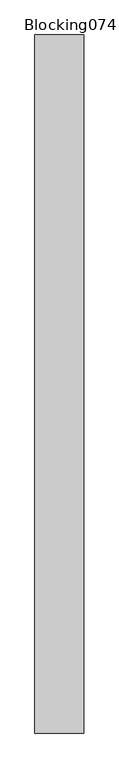
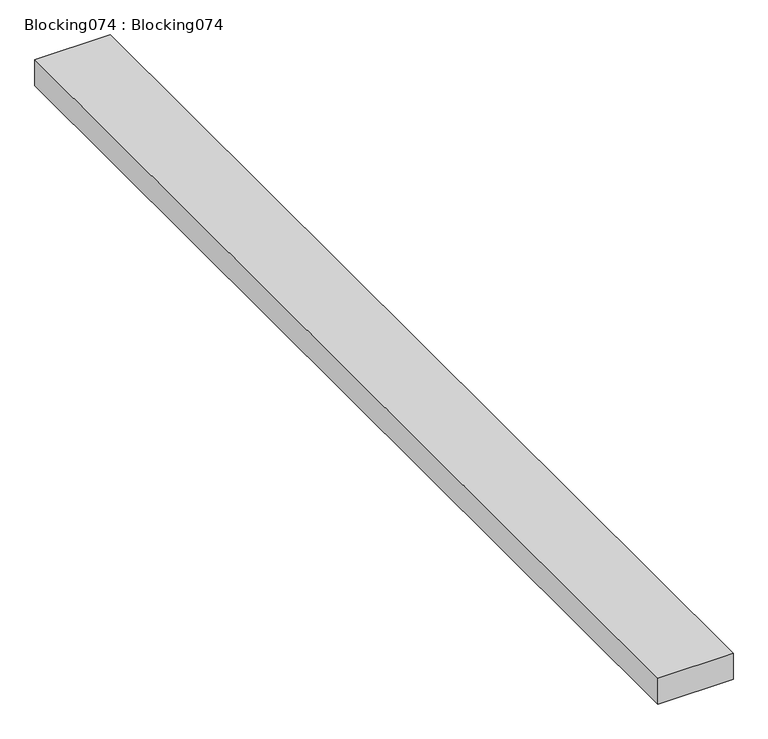
"""IFC4 building model written with IfcOpenShell, lengths in millimetres: proxy geometry, Blocking074 : Blocking074."""

import ifcopenshell
import ifcopenshell.guid

model = None  # the IFC model being written
_history = None  # IfcOwnerHistory: only IFC2X3 demands one
_inside = {}  # id of a spatial element -> (the spatial element, [elements in it])
_under = {}  # id of a project, library or spatial element -> (it, [spatial elements below it])
_declared = {}  # id of a project -> (the project, [libraries it declares])
_typed = {}  # id of a type object -> (the type object, [elements of that type])
_made_of = {}  # id of a material, layer set ... -> (it, [elements and type objects made of it])


def new_model(schema):
    """Start an empty IFC model of exactly this schema.

    Asked for "IFC4X3", IfcOpenShell would pick the latest addendum, in which some entities
    have other attributes; the version numbers below select the first issue.
    IFC2X3 requires an IfcOwnerHistory on every rooted entity: one is made here for all.
    """
    global model, _history
    if schema == "IFC4X3":
        model = ifcopenshell.file(schema_version=(4, 3, 0, 0))
    else:
        model = ifcopenshell.file(schema=schema)
    _inside.clear()
    _under.clear()
    _declared.clear()
    _typed.clear()
    _made_of.clear()
    _history = None
    if model.schema == "IFC2X3":
        org = make("IfcOrganization", Name="unknown")
        user = make(
            "IfcPersonAndOrganization",
            ThePerson=make("IfcPerson", FamilyName="unknown"),
            TheOrganization=org,
        )
        app = make(
            "IfcApplication",
            ApplicationDeveloper=org,
            Version="unknown",
            ApplicationFullName="unknown",
            ApplicationIdentifier="unknown",
        )
        _history = make(
            "IfcOwnerHistory",
            OwningUser=user,
            OwningApplication=app,
            ChangeAction="ADDED",
            CreationDate=0,
        )
    return model


def make(cls, **values):
    """One entity of the class cls with the attributes given. An attribute that is None is left unset."""
    return model.create_entity(
        cls, **{name: value for name, value in values.items() if value is not None}
    )


def rooted(cls, **values):
    """An entity with a GlobalId (a new one), such as an element, a storey or a relation."""
    return make(cls, GlobalId=ifcopenshell.guid.new(), OwnerHistory=_history, **values)


def si_unit(unit_type, name, prefix=None):
    """IfcSIUnit, for example si_unit("LENGTHUNIT", "METRE", prefix="MILLI")."""
    return make("IfcSIUnit", UnitType=unit_type, Prefix=prefix, Name=name)


def assignment(units):
    """IfcUnitAssignment: the units of a project."""
    return None if units is None else make("IfcUnitAssignment", Units=units)


def point(xyz):
    """IfcCartesianPoint."""
    return None if xyz is None else make("IfcCartesianPoint", Coordinates=xyz)


def direction(xyz):
    """IfcDirection."""
    return None if xyz is None else make("IfcDirection", DirectionRatios=xyz)


def frame(location, z_axis=None, x_axis=None):
    """IfcAxis2Placement3D, a coordinate frame: its origin and axes. An axis left out is left unset."""
    return make(
        "IfcAxis2Placement3D",
        Location=point(location),
        Axis=direction(z_axis),
        RefDirection=direction(x_axis),
    )


def origin():
    """The frame at (0, 0, 0) with its axes left unset."""
    return frame((0.0, 0.0, 0.0))


def place(relative_to, where):
    """IfcLocalPlacement: puts the frame where relative to a parent placement (None: the world)."""
    return make(
        "IfcLocalPlacement", PlacementRelTo=relative_to, RelativePlacement=where
    )


def context(
    kind, dimensions, precision=None, world=None, true_north=None, identifier=None
):
    """IfcGeometricRepresentationContext, for example the 3D "Model" context."""
    return make(
        "IfcGeometricRepresentationContext",
        ContextIdentifier=identifier,
        ContextType=kind,
        CoordinateSpaceDimension=dimensions,
        Precision=precision,
        WorldCoordinateSystem=world,
        TrueNorth=true_north,
    )


def project(units=None, contexts=None):
    """IfcProject with its units and contexts."""
    return rooted(
        "IfcProject",
        Name="project",
        RepresentationContexts=contexts,
        UnitsInContext=assignment(units),
    )


def spatial(cls, under=None, at=None, **own):
    """A site, building, storey or space (cls), placed at a placement, below another one or the project."""
    s = rooted(cls, ObjectPlacement=at, **own)
    if under is not None:
        _under.setdefault(under.id(), (under, []))[1].append(s)
    return s


def polyline(points):
    """IfcPolyline through the points."""
    return make("IfcPolyline", Points=[point(p) for p in points])


def outline(outer, holes=None, kind="AREA"):
    """IfcArbitraryClosedProfileDef: a profile drawn as a closed curve; with holes, ...WithVoids."""
    if holes is None:
        return make("IfcArbitraryClosedProfileDef", ProfileType=kind, OuterCurve=outer)
    return make(
        "IfcArbitraryProfileDefWithVoids",
        ProfileType=kind,
        OuterCurve=outer,
        InnerCurves=holes,
    )


def extrude(swept, where, along, depth):
    """IfcExtrudedAreaSolid: the profile swept, set in the frame where, extruded along a direction by depth."""
    return make(
        "IfcExtrudedAreaSolid",
        SweptArea=swept,
        Position=where,
        ExtrudedDirection=direction(along),
        Depth=depth,
    )


def shape(context_of_items, identifier, shape_type, items):
    """IfcShapeRepresentation: the items that make up one representation, for example the "Body"."""
    return make(
        "IfcShapeRepresentation",
        ContextOfItems=context_of_items,
        RepresentationIdentifier=identifier,
        RepresentationType=shape_type,
        Items=items,
    )


def source(mapping_origin, context_of_items, identifier, shape_type, items):
    """IfcRepresentationMap: a shape defined once, which mapped items show again and again."""
    return make(
        "IfcRepresentationMap",
        MappingOrigin=mapping_origin,
        MappedRepresentation=shape(context_of_items, identifier, shape_type, items),
    )


def transform(
    local_origin,
    x_axis=None,
    y_axis=None,
    z_axis=None,
    scale=None,
    scale2=None,
    scale3=None,
    uniform=True,
):
    """IfcCartesianTransformationOperator3D, or its non-uniform kind. x_axis, y_axis, z_axis: its Axis1, 2, 3."""
    if uniform:
        return make(
            "IfcCartesianTransformationOperator3D",
            Axis1=direction(x_axis),
            Axis2=direction(y_axis),
            LocalOrigin=point(local_origin),
            Scale=scale,
            Axis3=direction(z_axis),
        )
    return make(
        "IfcCartesianTransformationOperator3DnonUniform",
        Axis1=direction(x_axis),
        Axis2=direction(y_axis),
        LocalOrigin=point(local_origin),
        Scale=scale,
        Axis3=direction(z_axis),
        Scale2=scale2,
        Scale3=scale3,
    )


def mapped(mapping_source, mapping_target):
    """IfcMappedItem: shows the shape of a source again, moved by a transform."""
    return make(
        "IfcMappedItem", MappingSource=mapping_source, MappingTarget=mapping_target
    )


def made_of(thing, what):
    """Note that an element or type object is made of a material, layer set ...; save() writes the relation."""
    if what is not None:
        _made_of.setdefault(what.id(), (what, []))[1].append(thing)
    return thing


def element(
    cls,
    number,
    at=None,
    inside=None,
    cuts=None,
    type_object=None,
    material=None,
    context=None,
    identifier="Body",
    shape_type=None,
    held_by="IfcProductDefinitionShape",
    body=None,
    shapes=None,
    **own,
):
    """One element of the class cls, such as IfcWall. Its Tag is "e" and its number.

    at: its placement. inside: the storey or other place that contains it. cuts: it is an
    opening in that element (IfcRelVoidsElement). A single representation is given by context,
    identifier, shape_type and body (its items); several are given by shapes. held_by: the class
    of the entity that holds the representations. save() writes the other relations.
    """
    e = rooted(cls, Tag="e%d" % number, ObjectPlacement=at, **own)
    if body is not None:
        shapes = [shape(context, identifier, shape_type, body)]
    if shapes is not None:
        e.Representation = make(held_by, Representations=shapes)
    if inside is not None:
        _inside.setdefault(inside.id(), (inside, []))[1].append(e)
    if cuts is not None:
        rooted(
            "IfcRelVoidsElement", RelatingBuildingElement=cuts, RelatedOpeningElement=e
        )
    if type_object is not None:
        _typed.setdefault(type_object.id(), (type_object, []))[1].append(e)
    return made_of(e, material)


def aggregate(whole, parts):
    """IfcRelAggregates: a whole, such as a stair, and the parts it consists of."""
    return rooted("IfcRelAggregates", RelatingObject=whole, RelatedObjects=parts)


def save(model, path):
    """Write the relations noted so far, then the file.

    IfcRelAggregates (storeys below a building ...), IfcRelContainedInSpatialStructure (elements
    in a storey), IfcRelDefinesByType, IfcRelAssociatesMaterial and IfcRelDeclares: one each for
    every whole, place, type object, material and project.
    """
    for whole, parts in _under.values():
        aggregate(whole, parts)
    for where, things in _inside.values():
        rooted(
            "IfcRelContainedInSpatialStructure",
            RelatedElements=things,
            RelatingStructure=where,
        )
    for kind, things in _typed.values():
        rooted("IfcRelDefinesByType", RelatedObjects=things, RelatingType=kind)
    for what, things in _made_of.values():
        rooted("IfcRelAssociatesMaterial", RelatedObjects=things, RelatingMaterial=what)
    for by, libraries in _declared.values():
        rooted("IfcRelDeclares", RelatingContext=by, RelatedDefinitions=libraries)
    model.write(path)


def blocking074_blocking074_4a3d536d(model_context):
    return source(origin(), model_context, "Body", "SweptSolid", [
        extrude(outline(polyline([(-950.3815411, -1052.8908906), (-1090.0815411, -1052.8908906), (-1090.0815411, 947.1091094), (-950.3815411, 947.1091094), (-950.3815411, -1052.8908906)])), frame((0.0, 0.0, 40265.096), z_axis=(0.0, 0.0, 1.0), x_axis=(1.0, 0.0, 0.0)), (0.0, 0.0, 1.0), 50.8),
    ])


if __name__ == "__main__":
    model = new_model("IFC4")
    model_context = context("Model", 3, world=origin())
    ifc_project = project(units=[si_unit("LENGTHUNIT", "METRE", prefix="MILLI")], contexts=[model_context])
    site = spatial("IfcSite", under=ifc_project)
    building = spatial("IfcBuilding", under=site)
    placement = place(None, origin())
    blocking074_blocking074_shape = blocking074_blocking074_4a3d536d(model_context)
    element("IfcBuildingElementProxy", 1, Name="Blocking074 : Blocking074", ObjectType="Blocking074 : Blocking074", at=placement, inside=building, context=model_context, shape_type="MappedRepresentation", body=[
        mapped(blocking074_blocking074_shape, transform((0.0, 0.0, 0.0), x_axis=(1.0, 0.0, 0.0), y_axis=(0.0, 1.0, 0.0), z_axis=(0.0, 0.0, 1.0))),
    ])
    save(model, "model.ifc")

# Revit data of these elements
# Type "Blocking074 : Blocking074"
#   NameOverride = "Blocking074"
# Element 1 (IfcBuildingElementProxy, "Blocking074 : Blocking074")
#   Materials on its faces: "WOOD BLOCKING AS REQUIRED"
# Materials
#   "WOOD BLOCKING AS REQUIRED": class "Unassigned", colour RGB 166 124 85, transparency 0, Cost = 0
